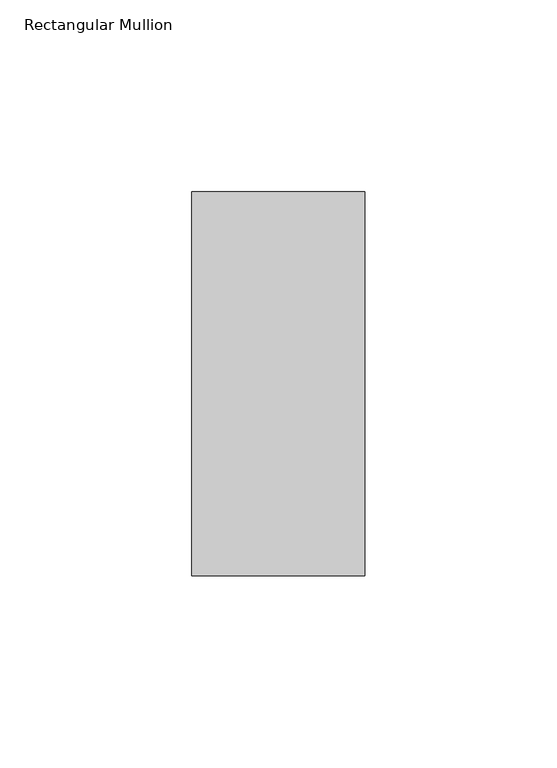
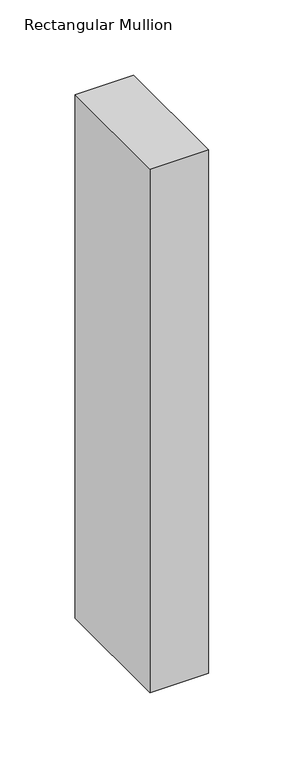
"""IFC4 building model written with IfcOpenShell, lengths in millimetres: member geometry, Rectangular Mullion : 알루미늄_Rectangular Cap_100 x 45."""

from ifc_helpers import new_model, si_unit, frame, origin, place, context, project, spatial, polyline, outline, extrude, source, transform, mapped, element, save


def rectangular_mullion_4dad3324(model_context):
    return source(origin(), model_context, "Body", "SweptSolid", [
        extrude(outline(polyline([(0.0, 50.0), (0.0, -50.0), (-45.0, -50.0), (-45.0, 50.0), (0.0, 50.0)])), frame((0.0, 0.0, -425.0), z_axis=(0.0, 0.0, 1.0), x_axis=(1.0, 0.0, 0.0)), (0.0, 0.0, 1.0), 425.0),
    ])


if __name__ == "__main__":
    model = new_model("IFC4")
    model_context = context("Model", 3, world=origin())
    ifc_project = project(units=[si_unit("LENGTHUNIT", "METRE", prefix="MILLI")], contexts=[model_context])
    site = spatial("IfcSite", under=ifc_project)
    building = spatial("IfcBuilding", under=site)
    placement = place(None, origin())
    rectangular_mullion_shape = rectangular_mullion_4dad3324(model_context)
    element("IfcMember", 1, ObjectType="Rectangular Mullion : 알루미늄_Rectangular Cap_100 x 45", at=placement, inside=building, context=model_context, shape_type="MappedRepresentation", body=[
        mapped(rectangular_mullion_shape, transform((0.0, 0.0, 0.0), x_axis=(1.0, 0.0, 0.0), y_axis=(0.0, 1.0, 0.0), z_axis=(0.0, 0.0, 1.0))),
    ])
    save(model, "model.ifc")

# Revit data of these elements
# Type "Rectangular Mullion : 알루미늄_Rectangular Cap_100 x 45"
#   built-in parameter 1007304 = 0.328084 (stored number, unit not read)
#   built-in parameter 1007301 = 0.0738189 (stored number, unit not read)
#   built-in parameter 1007300 = 0.0738189 (stored number, unit not read)
# Element 1 (IfcMember, "Rectangular Mullion : 알루미늄_Rectangular Cap_100 x 45")
#   Materials on its faces: "00_Metal_Stainless Steel"
# Materials
#   "00_Metal_Stainless Steel": class "Metal", colour RGB 148 148 148, transparency 0, Description = "Steel", Cost = 0
